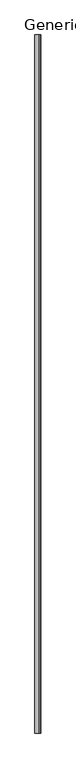
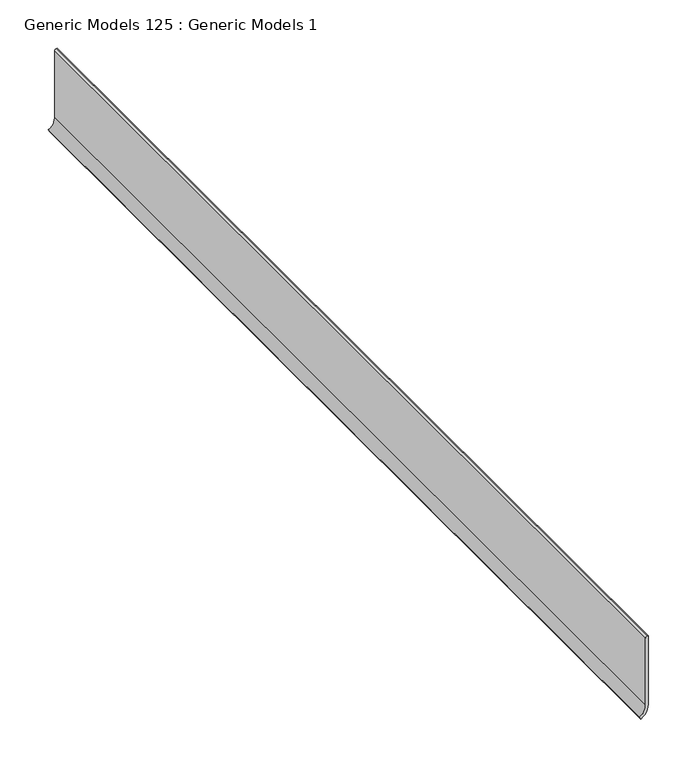
"""IFC4 building model written with IfcOpenShell, lengths in millimetres: proxy geometry, Generic Models 125 : Generic Models 1."""

import ifcopenshell
import ifcopenshell.guid

model = None  # the IFC model being written
_history = None  # IfcOwnerHistory: only IFC2X3 demands one
_inside = {}  # id of a spatial element -> (the spatial element, [elements in it])
_under = {}  # id of a project, library or spatial element -> (it, [spatial elements below it])
_declared = {}  # id of a project -> (the project, [libraries it declares])
_typed = {}  # id of a type object -> (the type object, [elements of that type])
_made_of = {}  # id of a material, layer set ... -> (it, [elements and type objects made of it])


def new_model(schema):
    """Start an empty IFC model of exactly this schema.

    Asked for "IFC4X3", IfcOpenShell would pick the latest addendum, in which some entities
    have other attributes; the version numbers below select the first issue.
    IFC2X3 requires an IfcOwnerHistory on every rooted entity: one is made here for all.
    """
    global model, _history
    if schema == "IFC4X3":
        model = ifcopenshell.file(schema_version=(4, 3, 0, 0))
    else:
        model = ifcopenshell.file(schema=schema)
    _inside.clear()
    _under.clear()
    _declared.clear()
    _typed.clear()
    _made_of.clear()
    _history = None
    if model.schema == "IFC2X3":
        org = make("IfcOrganization", Name="unknown")
        user = make(
            "IfcPersonAndOrganization",
            ThePerson=make("IfcPerson", FamilyName="unknown"),
            TheOrganization=org,
        )
        app = make(
            "IfcApplication",
            ApplicationDeveloper=org,
            Version="unknown",
            ApplicationFullName="unknown",
            ApplicationIdentifier="unknown",
        )
        _history = make(
            "IfcOwnerHistory",
            OwningUser=user,
            OwningApplication=app,
            ChangeAction="ADDED",
            CreationDate=0,
        )
    return model


def make(cls, **values):
    """One entity of the class cls with the attributes given. An attribute that is None is left unset."""
    return model.create_entity(
        cls, **{name: value for name, value in values.items() if value is not None}
    )


def rooted(cls, **values):
    """An entity with a GlobalId (a new one), such as an element, a storey or a relation."""
    return make(cls, GlobalId=ifcopenshell.guid.new(), OwnerHistory=_history, **values)


def si_unit(unit_type, name, prefix=None):
    """IfcSIUnit, for example si_unit("LENGTHUNIT", "METRE", prefix="MILLI")."""
    return make("IfcSIUnit", UnitType=unit_type, Prefix=prefix, Name=name)


def assignment(units):
    """IfcUnitAssignment: the units of a project."""
    return None if units is None else make("IfcUnitAssignment", Units=units)


def point(xyz):
    """IfcCartesianPoint."""
    return None if xyz is None else make("IfcCartesianPoint", Coordinates=xyz)


def direction(xyz):
    """IfcDirection."""
    return None if xyz is None else make("IfcDirection", DirectionRatios=xyz)


def frame(location, z_axis=None, x_axis=None):
    """IfcAxis2Placement3D, a coordinate frame: its origin and axes. An axis left out is left unset."""
    return make(
        "IfcAxis2Placement3D",
        Location=point(location),
        Axis=direction(z_axis),
        RefDirection=direction(x_axis),
    )


def frame_2d(location, x_axis=None):
    """IfcAxis2Placement2D, a coordinate frame in the plane: its origin and x axis."""
    return make(
        "IfcAxis2Placement2D", Location=point(location), RefDirection=direction(x_axis)
    )


def origin():
    """The frame at (0, 0, 0) with its axes left unset."""
    return frame((0.0, 0.0, 0.0))


def place(relative_to, where):
    """IfcLocalPlacement: puts the frame where relative to a parent placement (None: the world)."""
    return make(
        "IfcLocalPlacement", PlacementRelTo=relative_to, RelativePlacement=where
    )


def context(
    kind, dimensions, precision=None, world=None, true_north=None, identifier=None
):
    """IfcGeometricRepresentationContext, for example the 3D "Model" context."""
    return make(
        "IfcGeometricRepresentationContext",
        ContextIdentifier=identifier,
        ContextType=kind,
        CoordinateSpaceDimension=dimensions,
        Precision=precision,
        WorldCoordinateSystem=world,
        TrueNorth=true_north,
    )


def project(units=None, contexts=None):
    """IfcProject with its units and contexts."""
    return rooted(
        "IfcProject",
        Name="project",
        RepresentationContexts=contexts,
        UnitsInContext=assignment(units),
    )


def spatial(cls, under=None, at=None, **own):
    """A site, building, storey or space (cls), placed at a placement, below another one or the project."""
    s = rooted(cls, ObjectPlacement=at, **own)
    if under is not None:
        _under.setdefault(under.id(), (under, []))[1].append(s)
    return s


def polyline(points):
    """IfcPolyline through the points."""
    return make("IfcPolyline", Points=[point(p) for p in points])


def circle_curve(where, radius):
    """IfcCircle in the frame where."""
    return make("IfcCircle", Position=where, Radius=radius)


def trimmed(basis, trim1, trim2, sense, master):
    """IfcTrimmedCurve: the piece of a basis curve between two trims."""
    return make(
        "IfcTrimmedCurve",
        BasisCurve=basis,
        Trim1=trim1,
        Trim2=trim2,
        SenseAgreement=sense,
        MasterRepresentation=master,
    )


def segment(curve, same_sense, transition):
    """IfcCompositeCurveSegment."""
    return make(
        "IfcCompositeCurveSegment",
        Transition=transition,
        SameSense=same_sense,
        ParentCurve=curve,
    )


def composite_curve(segments, self_intersect=None):
    """IfcCompositeCurve: segments joined end to end."""
    return make("IfcCompositeCurve", Segments=segments, SelfIntersect=self_intersect)


def outline(outer, holes=None, kind="AREA"):
    """IfcArbitraryClosedProfileDef: a profile drawn as a closed curve; with holes, ...WithVoids."""
    if holes is None:
        return make("IfcArbitraryClosedProfileDef", ProfileType=kind, OuterCurve=outer)
    return make(
        "IfcArbitraryProfileDefWithVoids",
        ProfileType=kind,
        OuterCurve=outer,
        InnerCurves=holes,
    )


def extrude(swept, where, along, depth):
    """IfcExtrudedAreaSolid: the profile swept, set in the frame where, extruded along a direction by depth."""
    return make(
        "IfcExtrudedAreaSolid",
        SweptArea=swept,
        Position=where,
        ExtrudedDirection=direction(along),
        Depth=depth,
    )


def shape(context_of_items, identifier, shape_type, items):
    """IfcShapeRepresentation: the items that make up one representation, for example the "Body"."""
    return make(
        "IfcShapeRepresentation",
        ContextOfItems=context_of_items,
        RepresentationIdentifier=identifier,
        RepresentationType=shape_type,
        Items=items,
    )


def source(mapping_origin, context_of_items, identifier, shape_type, items):
    """IfcRepresentationMap: a shape defined once, which mapped items show again and again."""
    return make(
        "IfcRepresentationMap",
        MappingOrigin=mapping_origin,
        MappedRepresentation=shape(context_of_items, identifier, shape_type, items),
    )


def transform(
    local_origin,
    x_axis=None,
    y_axis=None,
    z_axis=None,
    scale=None,
    scale2=None,
    scale3=None,
    uniform=True,
):
    """IfcCartesianTransformationOperator3D, or its non-uniform kind. x_axis, y_axis, z_axis: its Axis1, 2, 3."""
    if uniform:
        return make(
            "IfcCartesianTransformationOperator3D",
            Axis1=direction(x_axis),
            Axis2=direction(y_axis),
            LocalOrigin=point(local_origin),
            Scale=scale,
            Axis3=direction(z_axis),
        )
    return make(
        "IfcCartesianTransformationOperator3DnonUniform",
        Axis1=direction(x_axis),
        Axis2=direction(y_axis),
        LocalOrigin=point(local_origin),
        Scale=scale,
        Axis3=direction(z_axis),
        Scale2=scale2,
        Scale3=scale3,
    )


def mapped(mapping_source, mapping_target):
    """IfcMappedItem: shows the shape of a source again, moved by a transform."""
    return make(
        "IfcMappedItem", MappingSource=mapping_source, MappingTarget=mapping_target
    )


def made_of(thing, what):
    """Note that an element or type object is made of a material, layer set ...; save() writes the relation."""
    if what is not None:
        _made_of.setdefault(what.id(), (what, []))[1].append(thing)
    return thing


def element(
    cls,
    number,
    at=None,
    inside=None,
    cuts=None,
    type_object=None,
    material=None,
    context=None,
    identifier="Body",
    shape_type=None,
    held_by="IfcProductDefinitionShape",
    body=None,
    shapes=None,
    **own,
):
    """One element of the class cls, such as IfcWall. Its Tag is "e" and its number.

    at: its placement. inside: the storey or other place that contains it. cuts: it is an
    opening in that element (IfcRelVoidsElement). A single representation is given by context,
    identifier, shape_type and body (its items); several are given by shapes. held_by: the class
    of the entity that holds the representations. save() writes the other relations.
    """
    e = rooted(cls, Tag="e%d" % number, ObjectPlacement=at, **own)
    if body is not None:
        shapes = [shape(context, identifier, shape_type, body)]
    if shapes is not None:
        e.Representation = make(held_by, Representations=shapes)
    if inside is not None:
        _inside.setdefault(inside.id(), (inside, []))[1].append(e)
    if cuts is not None:
        rooted(
            "IfcRelVoidsElement", RelatingBuildingElement=cuts, RelatedOpeningElement=e
        )
    if type_object is not None:
        _typed.setdefault(type_object.id(), (type_object, []))[1].append(e)
    return made_of(e, material)


def aggregate(whole, parts):
    """IfcRelAggregates: a whole, such as a stair, and the parts it consists of."""
    return rooted("IfcRelAggregates", RelatingObject=whole, RelatedObjects=parts)


def save(model, path):
    """Write the relations noted so far, then the file.

    IfcRelAggregates (storeys below a building ...), IfcRelContainedInSpatialStructure (elements
    in a storey), IfcRelDefinesByType, IfcRelAssociatesMaterial and IfcRelDeclares: one each for
    every whole, place, type object, material and project.
    """
    for whole, parts in _under.values():
        aggregate(whole, parts)
    for where, things in _inside.values():
        rooted(
            "IfcRelContainedInSpatialStructure",
            RelatedElements=things,
            RelatingStructure=where,
        )
    for kind, things in _typed.values():
        rooted("IfcRelDefinesByType", RelatedObjects=things, RelatingType=kind)
    for what, things in _made_of.values():
        rooted("IfcRelAssociatesMaterial", RelatedObjects=things, RelatingMaterial=what)
    for by, libraries in _declared.values():
        rooted("IfcRelDeclares", RelatingContext=by, RelatedDefinitions=libraries)
    model.write(path)


def generic_models_125_generic_models_1_5b15c746(model_context):
    return source(origin(), model_context, "Body", "SweptSolid", [
        extrude(outline(composite_curve([segment(polyline([(-124.376067, 46827.9235531), (-124.376067, 46826.8353549)]), True, "CONTINUOUS"), segment(trimmed(circle_curve(frame_2d((-126.4628688, 46826.8353549)), 2.0868018), [point((-124.376067, 46826.8353549))], [point((-126.4628688, 46824.7485531))], False, "CARTESIAN"), True, "CONTINUOUS"), segment(polyline([(-126.4628688, 46824.7485531), (-210.5264363, 46824.7485531)]), True, "CONTINUOUS"), segment(trimmed(circle_curve(frame_2d((-210.5264363, 46810.0838562)), 14.6646968), [point((-210.5264363, 46824.7485531))], [point((-223.2264363, 46817.4162046))], True, "CARTESIAN"), True, "CONTINUOUS"), segment(polyline([(-223.2264363, 46817.4162046), (-225.976067, 46819.0037046)]), True, "CONTINUOUS"), segment(trimmed(circle_curve(frame_2d((-210.5264363, 46810.0838562)), 17.8396968), [point((-225.976067, 46819.0037046))], [point((-210.5264363, 46827.9235531))], False, "CARTESIAN"), True, "CONTINUOUS"), segment(polyline([(-210.5264363, 46827.9235531), (-124.376067, 46827.9235531)]), True, "CONTINUOUS")], self_intersect=False)), frame((0.0, 0.0, 0.0), z_axis=(0.0, 1.0, 0.0), x_axis=(0.0, 0.0, 1.0)), (0.0, 0.0, 1.0), 1219.2),
    ])


if __name__ == "__main__":
    model = new_model("IFC4")
    model_context = context("Model", 3, world=origin())
    ifc_project = project(units=[si_unit("LENGTHUNIT", "METRE", prefix="MILLI")], contexts=[model_context])
    site = spatial("IfcSite", under=ifc_project)
    building = spatial("IfcBuilding", under=site)
    placement = place(None, origin())
    generic_models_125_generic_models_1_shape = generic_models_125_generic_models_1_5b15c746(model_context)
    element("IfcBuildingElementProxy", 1, Name="Generic Models 125 : Generic Models 1", ObjectType="Generic Models 125 : Generic Models 1", at=placement, inside=building, context=model_context, shape_type="MappedRepresentation", body=[
        mapped(generic_models_125_generic_models_1_shape, transform((0.0, 0.0, 0.0), x_axis=(1.0, 0.0, 0.0), y_axis=(0.0, 1.0, 0.0), z_axis=(0.0, 0.0, 1.0))),
    ])
    save(model, "model.ifc")

# Revit data of these elements
# Element 1 (IfcBuildingElementProxy, "Generic Models 125 : Generic Models 1")
#   Materials on its faces: "MATCH EXISTING BASE"
# Materials
#   "MATCH EXISTING BASE": class "Generic", colour RGB 120 120 120, transparency 0, Cost = 0
